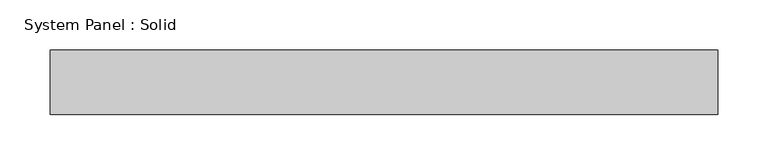
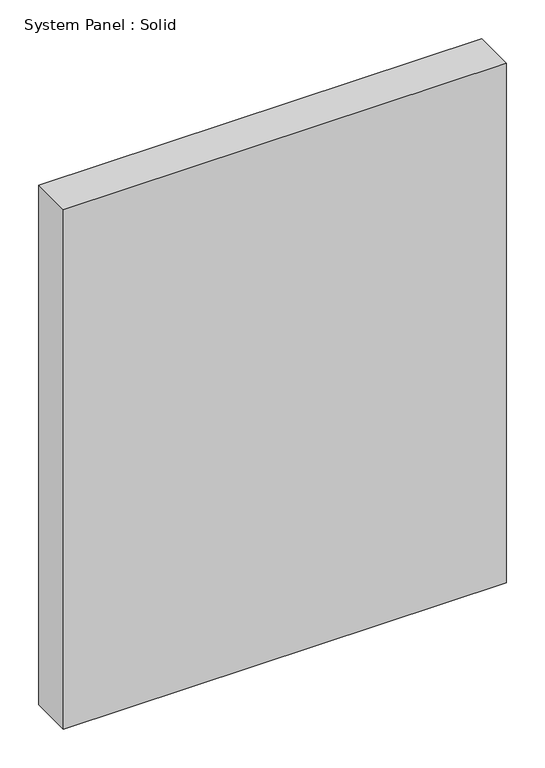
"""IFC4 building model written with IfcOpenShell, lengths in millimetres: plate geometry, System Panel : Solid."""

import ifcopenshell
import ifcopenshell.guid

model = None  # the IFC model being written
_history = None  # IfcOwnerHistory: only IFC2X3 demands one
_inside = {}  # id of a spatial element -> (the spatial element, [elements in it])
_under = {}  # id of a project, library or spatial element -> (it, [spatial elements below it])
_declared = {}  # id of a project -> (the project, [libraries it declares])
_typed = {}  # id of a type object -> (the type object, [elements of that type])
_made_of = {}  # id of a material, layer set ... -> (it, [elements and type objects made of it])


def new_model(schema):
    """Start an empty IFC model of exactly this schema.

    Asked for "IFC4X3", IfcOpenShell would pick the latest addendum, in which some entities
    have other attributes; the version numbers below select the first issue.
    IFC2X3 requires an IfcOwnerHistory on every rooted entity: one is made here for all.
    """
    global model, _history
    if schema == "IFC4X3":
        model = ifcopenshell.file(schema_version=(4, 3, 0, 0))
    else:
        model = ifcopenshell.file(schema=schema)
    _inside.clear()
    _under.clear()
    _declared.clear()
    _typed.clear()
    _made_of.clear()
    _history = None
    if model.schema == "IFC2X3":
        org = make("IfcOrganization", Name="unknown")
        user = make(
            "IfcPersonAndOrganization",
            ThePerson=make("IfcPerson", FamilyName="unknown"),
            TheOrganization=org,
        )
        app = make(
            "IfcApplication",
            ApplicationDeveloper=org,
            Version="unknown",
            ApplicationFullName="unknown",
            ApplicationIdentifier="unknown",
        )
        _history = make(
            "IfcOwnerHistory",
            OwningUser=user,
            OwningApplication=app,
            ChangeAction="ADDED",
            CreationDate=0,
        )
    return model


def make(cls, **values):
    """One entity of the class cls with the attributes given. An attribute that is None is left unset."""
    return model.create_entity(
        cls, **{name: value for name, value in values.items() if value is not None}
    )


def rooted(cls, **values):
    """An entity with a GlobalId (a new one), such as an element, a storey or a relation."""
    return make(cls, GlobalId=ifcopenshell.guid.new(), OwnerHistory=_history, **values)


def si_unit(unit_type, name, prefix=None):
    """IfcSIUnit, for example si_unit("LENGTHUNIT", "METRE", prefix="MILLI")."""
    return make("IfcSIUnit", UnitType=unit_type, Prefix=prefix, Name=name)


def assignment(units):
    """IfcUnitAssignment: the units of a project."""
    return None if units is None else make("IfcUnitAssignment", Units=units)


def point(xyz):
    """IfcCartesianPoint."""
    return None if xyz is None else make("IfcCartesianPoint", Coordinates=xyz)


def direction(xyz):
    """IfcDirection."""
    return None if xyz is None else make("IfcDirection", DirectionRatios=xyz)


def frame(location, z_axis=None, x_axis=None):
    """IfcAxis2Placement3D, a coordinate frame: its origin and axes. An axis left out is left unset."""
    return make(
        "IfcAxis2Placement3D",
        Location=point(location),
        Axis=direction(z_axis),
        RefDirection=direction(x_axis),
    )


def origin():
    """The frame at (0, 0, 0) with its axes left unset."""
    return frame((0.0, 0.0, 0.0))


def origin_with_axes():
    """The frame at (0, 0, 0) with the z axis (0, 0, 1) and the x axis (1, 0, 0) written out."""
    return frame((0.0, 0.0, 0.0), z_axis=(0.0, 0.0, 1.0), x_axis=(1.0, 0.0, 0.0))


def place(relative_to, where):
    """IfcLocalPlacement: puts the frame where relative to a parent placement (None: the world)."""
    return make(
        "IfcLocalPlacement", PlacementRelTo=relative_to, RelativePlacement=where
    )


def context(
    kind, dimensions, precision=None, world=None, true_north=None, identifier=None
):
    """IfcGeometricRepresentationContext, for example the 3D "Model" context."""
    return make(
        "IfcGeometricRepresentationContext",
        ContextIdentifier=identifier,
        ContextType=kind,
        CoordinateSpaceDimension=dimensions,
        Precision=precision,
        WorldCoordinateSystem=world,
        TrueNorth=true_north,
    )


def project(units=None, contexts=None):
    """IfcProject with its units and contexts."""
    return rooted(
        "IfcProject",
        Name="project",
        RepresentationContexts=contexts,
        UnitsInContext=assignment(units),
    )


def spatial(cls, under=None, at=None, **own):
    """A site, building, storey or space (cls), placed at a placement, below another one or the project."""
    s = rooted(cls, ObjectPlacement=at, **own)
    if under is not None:
        _under.setdefault(under.id(), (under, []))[1].append(s)
    return s


def polyline(points):
    """IfcPolyline through the points."""
    return make("IfcPolyline", Points=[point(p) for p in points])


def outline(outer, holes=None, kind="AREA"):
    """IfcArbitraryClosedProfileDef: a profile drawn as a closed curve; with holes, ...WithVoids."""
    if holes is None:
        return make("IfcArbitraryClosedProfileDef", ProfileType=kind, OuterCurve=outer)
    return make(
        "IfcArbitraryProfileDefWithVoids",
        ProfileType=kind,
        OuterCurve=outer,
        InnerCurves=holes,
    )


def extrude(swept, where, along, depth):
    """IfcExtrudedAreaSolid: the profile swept, set in the frame where, extruded along a direction by depth."""
    return make(
        "IfcExtrudedAreaSolid",
        SweptArea=swept,
        Position=where,
        ExtrudedDirection=direction(along),
        Depth=depth,
    )


def shape(context_of_items, identifier, shape_type, items):
    """IfcShapeRepresentation: the items that make up one representation, for example the "Body"."""
    return make(
        "IfcShapeRepresentation",
        ContextOfItems=context_of_items,
        RepresentationIdentifier=identifier,
        RepresentationType=shape_type,
        Items=items,
    )


def source(mapping_origin, context_of_items, identifier, shape_type, items):
    """IfcRepresentationMap: a shape defined once, which mapped items show again and again."""
    return make(
        "IfcRepresentationMap",
        MappingOrigin=mapping_origin,
        MappedRepresentation=shape(context_of_items, identifier, shape_type, items),
    )


def transform(
    local_origin,
    x_axis=None,
    y_axis=None,
    z_axis=None,
    scale=None,
    scale2=None,
    scale3=None,
    uniform=True,
):
    """IfcCartesianTransformationOperator3D, or its non-uniform kind. x_axis, y_axis, z_axis: its Axis1, 2, 3."""
    if uniform:
        return make(
            "IfcCartesianTransformationOperator3D",
            Axis1=direction(x_axis),
            Axis2=direction(y_axis),
            LocalOrigin=point(local_origin),
            Scale=scale,
            Axis3=direction(z_axis),
        )
    return make(
        "IfcCartesianTransformationOperator3DnonUniform",
        Axis1=direction(x_axis),
        Axis2=direction(y_axis),
        LocalOrigin=point(local_origin),
        Scale=scale,
        Axis3=direction(z_axis),
        Scale2=scale2,
        Scale3=scale3,
    )


def mapped(mapping_source, mapping_target):
    """IfcMappedItem: shows the shape of a source again, moved by a transform."""
    return make(
        "IfcMappedItem", MappingSource=mapping_source, MappingTarget=mapping_target
    )


def made_of(thing, what):
    """Note that an element or type object is made of a material, layer set ...; save() writes the relation."""
    if what is not None:
        _made_of.setdefault(what.id(), (what, []))[1].append(thing)
    return thing


def element(
    cls,
    number,
    at=None,
    inside=None,
    cuts=None,
    type_object=None,
    material=None,
    context=None,
    identifier="Body",
    shape_type=None,
    held_by="IfcProductDefinitionShape",
    body=None,
    shapes=None,
    **own,
):
    """One element of the class cls, such as IfcWall. Its Tag is "e" and its number.

    at: its placement. inside: the storey or other place that contains it. cuts: it is an
    opening in that element (IfcRelVoidsElement). A single representation is given by context,
    identifier, shape_type and body (its items); several are given by shapes. held_by: the class
    of the entity that holds the representations. save() writes the other relations.
    """
    e = rooted(cls, Tag="e%d" % number, ObjectPlacement=at, **own)
    if body is not None:
        shapes = [shape(context, identifier, shape_type, body)]
    if shapes is not None:
        e.Representation = make(held_by, Representations=shapes)
    if inside is not None:
        _inside.setdefault(inside.id(), (inside, []))[1].append(e)
    if cuts is not None:
        rooted(
            "IfcRelVoidsElement", RelatingBuildingElement=cuts, RelatedOpeningElement=e
        )
    if type_object is not None:
        _typed.setdefault(type_object.id(), (type_object, []))[1].append(e)
    return made_of(e, material)


def aggregate(whole, parts):
    """IfcRelAggregates: a whole, such as a stair, and the parts it consists of."""
    return rooted("IfcRelAggregates", RelatingObject=whole, RelatedObjects=parts)


def save(model, path):
    """Write the relations noted so far, then the file.

    IfcRelAggregates (storeys below a building ...), IfcRelContainedInSpatialStructure (elements
    in a storey), IfcRelDefinesByType, IfcRelAssociatesMaterial and IfcRelDeclares: one each for
    every whole, place, type object, material and project.
    """
    for whole, parts in _under.values():
        aggregate(whole, parts)
    for where, things in _inside.values():
        rooted(
            "IfcRelContainedInSpatialStructure",
            RelatedElements=things,
            RelatingStructure=where,
        )
    for kind, things in _typed.values():
        rooted("IfcRelDefinesByType", RelatedObjects=things, RelatingType=kind)
    for what, things in _made_of.values():
        rooted("IfcRelAssociatesMaterial", RelatedObjects=things, RelatingMaterial=what)
    for by, libraries in _declared.values():
        rooted("IfcRelDeclares", RelatingContext=by, RelatedDefinitions=libraries)
    model.write(path)


def system_panel_solid_90d8cc78(model_context):
    return source(origin(), model_context, "Body", "SweptSolid", [
        extrude(outline(polyline([(330.2, -44.45), (-330.2, -44.45), (-330.2, 19.05), (330.2, 19.05), (330.2, -44.45)])), origin_with_axes(), (0.0, 0.0, 1.0), 819.15),
    ])


if __name__ == "__main__":
    model = new_model("IFC4")
    model_context = context("Model", 3, world=origin())
    ifc_project = project(units=[si_unit("LENGTHUNIT", "METRE", prefix="MILLI")], contexts=[model_context])
    site = spatial("IfcSite", under=ifc_project)
    building = spatial("IfcBuilding", under=site)
    placement = place(None, origin())
    system_panel_solid_shape = system_panel_solid_90d8cc78(model_context)
    element("IfcPlate", 1, ObjectType="System Panel : Solid", at=placement, inside=building, context=model_context, shape_type="MappedRepresentation", body=[
        mapped(system_panel_solid_shape, transform((0.0, 0.0, 0.0), x_axis=(1.0, 0.0, 0.0), y_axis=(0.0, 1.0, 0.0), z_axis=(0.0, 0.0, 1.0))),
    ])
    save(model, "model.ifc")

# Revit data of these elements
# Type "System Panel : Solid"
#   Construction Type Id = "MDOOR"
#   Analytic Construction = "Metal"
#   Visual Light Transmittance = 0
#   Solar Heat Gain Coefficient = 0
#   Heat Transfer Coefficient (U) = 0.651978 BTU/(h·ft²·°F)
#   Define Thermal Properties by = 1
# Element 1 (IfcPlate, "System Panel : Solid")
#   Materials on its faces: "Default"
# Materials
#   "Default": class "Miscellaneous", colour RGB 127 127 127, transparency 0, Cost = 0
